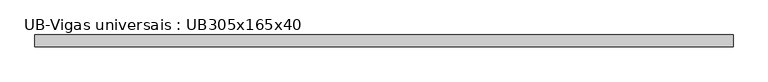
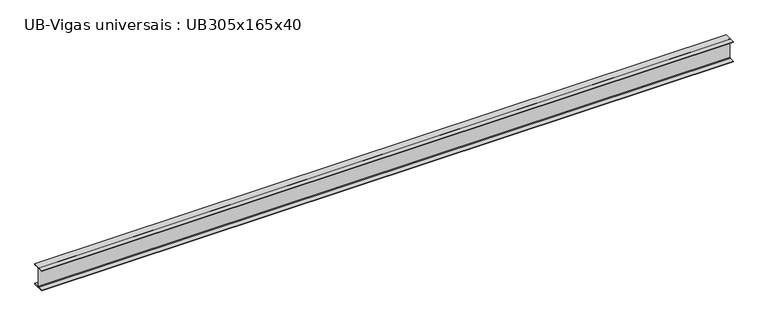
"""IFC4 building model written with IfcOpenShell, lengths in millimetres: beam geometry, UB-Vigas universais : UB305x165x40."""

import ifcopenshell
import ifcopenshell.guid

model = None  # the IFC model being written
_history = None  # IfcOwnerHistory: only IFC2X3 demands one
_inside = {}  # id of a spatial element -> (the spatial element, [elements in it])
_under = {}  # id of a project, library or spatial element -> (it, [spatial elements below it])
_declared = {}  # id of a project -> (the project, [libraries it declares])
_typed = {}  # id of a type object -> (the type object, [elements of that type])
_made_of = {}  # id of a material, layer set ... -> (it, [elements and type objects made of it])


def new_model(schema):
    """Start an empty IFC model of exactly this schema.

    Asked for "IFC4X3", IfcOpenShell would pick the latest addendum, in which some entities
    have other attributes; the version numbers below select the first issue.
    IFC2X3 requires an IfcOwnerHistory on every rooted entity: one is made here for all.
    """
    global model, _history
    if schema == "IFC4X3":
        model = ifcopenshell.file(schema_version=(4, 3, 0, 0))
    else:
        model = ifcopenshell.file(schema=schema)
    _inside.clear()
    _under.clear()
    _declared.clear()
    _typed.clear()
    _made_of.clear()
    _history = None
    if model.schema == "IFC2X3":
        org = make("IfcOrganization", Name="unknown")
        user = make(
            "IfcPersonAndOrganization",
            ThePerson=make("IfcPerson", FamilyName="unknown"),
            TheOrganization=org,
        )
        app = make(
            "IfcApplication",
            ApplicationDeveloper=org,
            Version="unknown",
            ApplicationFullName="unknown",
            ApplicationIdentifier="unknown",
        )
        _history = make(
            "IfcOwnerHistory",
            OwningUser=user,
            OwningApplication=app,
            ChangeAction="ADDED",
            CreationDate=0,
        )
    return model


def make(cls, **values):
    """One entity of the class cls with the attributes given. An attribute that is None is left unset."""
    return model.create_entity(
        cls, **{name: value for name, value in values.items() if value is not None}
    )


def rooted(cls, **values):
    """An entity with a GlobalId (a new one), such as an element, a storey or a relation."""
    return make(cls, GlobalId=ifcopenshell.guid.new(), OwnerHistory=_history, **values)


def si_unit(unit_type, name, prefix=None):
    """IfcSIUnit, for example si_unit("LENGTHUNIT", "METRE", prefix="MILLI")."""
    return make("IfcSIUnit", UnitType=unit_type, Prefix=prefix, Name=name)


def assignment(units):
    """IfcUnitAssignment: the units of a project."""
    return None if units is None else make("IfcUnitAssignment", Units=units)


def point(xyz):
    """IfcCartesianPoint."""
    return None if xyz is None else make("IfcCartesianPoint", Coordinates=xyz)


def direction(xyz):
    """IfcDirection."""
    return None if xyz is None else make("IfcDirection", DirectionRatios=xyz)


def frame(location, z_axis=None, x_axis=None):
    """IfcAxis2Placement3D, a coordinate frame: its origin and axes. An axis left out is left unset."""
    return make(
        "IfcAxis2Placement3D",
        Location=point(location),
        Axis=direction(z_axis),
        RefDirection=direction(x_axis),
    )


def frame_2d(location, x_axis=None):
    """IfcAxis2Placement2D, a coordinate frame in the plane: its origin and x axis."""
    return make(
        "IfcAxis2Placement2D", Location=point(location), RefDirection=direction(x_axis)
    )


def origin():
    """The frame at (0, 0, 0) with its axes left unset."""
    return frame((0.0, 0.0, 0.0))


def place(relative_to, where):
    """IfcLocalPlacement: puts the frame where relative to a parent placement (None: the world)."""
    return make(
        "IfcLocalPlacement", PlacementRelTo=relative_to, RelativePlacement=where
    )


def context(
    kind, dimensions, precision=None, world=None, true_north=None, identifier=None
):
    """IfcGeometricRepresentationContext, for example the 3D "Model" context."""
    return make(
        "IfcGeometricRepresentationContext",
        ContextIdentifier=identifier,
        ContextType=kind,
        CoordinateSpaceDimension=dimensions,
        Precision=precision,
        WorldCoordinateSystem=world,
        TrueNorth=true_north,
    )


def project(units=None, contexts=None):
    """IfcProject with its units and contexts."""
    return rooted(
        "IfcProject",
        Name="project",
        RepresentationContexts=contexts,
        UnitsInContext=assignment(units),
    )


def spatial(cls, under=None, at=None, **own):
    """A site, building, storey or space (cls), placed at a placement, below another one or the project."""
    s = rooted(cls, ObjectPlacement=at, **own)
    if under is not None:
        _under.setdefault(under.id(), (under, []))[1].append(s)
    return s


def polyline(points):
    """IfcPolyline through the points."""
    return make("IfcPolyline", Points=[point(p) for p in points])


def circle_curve(where, radius):
    """IfcCircle in the frame where."""
    return make("IfcCircle", Position=where, Radius=radius)


def trimmed(basis, trim1, trim2, sense, master):
    """IfcTrimmedCurve: the piece of a basis curve between two trims."""
    return make(
        "IfcTrimmedCurve",
        BasisCurve=basis,
        Trim1=trim1,
        Trim2=trim2,
        SenseAgreement=sense,
        MasterRepresentation=master,
    )


def segment(curve, same_sense, transition):
    """IfcCompositeCurveSegment."""
    return make(
        "IfcCompositeCurveSegment",
        Transition=transition,
        SameSense=same_sense,
        ParentCurve=curve,
    )


def composite_curve(segments, self_intersect=None):
    """IfcCompositeCurve: segments joined end to end."""
    return make("IfcCompositeCurve", Segments=segments, SelfIntersect=self_intersect)


def outline(outer, holes=None, kind="AREA"):
    """IfcArbitraryClosedProfileDef: a profile drawn as a closed curve; with holes, ...WithVoids."""
    if holes is None:
        return make("IfcArbitraryClosedProfileDef", ProfileType=kind, OuterCurve=outer)
    return make(
        "IfcArbitraryProfileDefWithVoids",
        ProfileType=kind,
        OuterCurve=outer,
        InnerCurves=holes,
    )


def extrude(swept, where, along, depth):
    """IfcExtrudedAreaSolid: the profile swept, set in the frame where, extruded along a direction by depth."""
    return make(
        "IfcExtrudedAreaSolid",
        SweptArea=swept,
        Position=where,
        ExtrudedDirection=direction(along),
        Depth=depth,
    )


def shape(context_of_items, identifier, shape_type, items):
    """IfcShapeRepresentation: the items that make up one representation, for example the "Body"."""
    return make(
        "IfcShapeRepresentation",
        ContextOfItems=context_of_items,
        RepresentationIdentifier=identifier,
        RepresentationType=shape_type,
        Items=items,
    )


def source(mapping_origin, context_of_items, identifier, shape_type, items):
    """IfcRepresentationMap: a shape defined once, which mapped items show again and again."""
    return make(
        "IfcRepresentationMap",
        MappingOrigin=mapping_origin,
        MappedRepresentation=shape(context_of_items, identifier, shape_type, items),
    )


def transform(
    local_origin,
    x_axis=None,
    y_axis=None,
    z_axis=None,
    scale=None,
    scale2=None,
    scale3=None,
    uniform=True,
):
    """IfcCartesianTransformationOperator3D, or its non-uniform kind. x_axis, y_axis, z_axis: its Axis1, 2, 3."""
    if uniform:
        return make(
            "IfcCartesianTransformationOperator3D",
            Axis1=direction(x_axis),
            Axis2=direction(y_axis),
            LocalOrigin=point(local_origin),
            Scale=scale,
            Axis3=direction(z_axis),
        )
    return make(
        "IfcCartesianTransformationOperator3DnonUniform",
        Axis1=direction(x_axis),
        Axis2=direction(y_axis),
        LocalOrigin=point(local_origin),
        Scale=scale,
        Axis3=direction(z_axis),
        Scale2=scale2,
        Scale3=scale3,
    )


def mapped(mapping_source, mapping_target):
    """IfcMappedItem: shows the shape of a source again, moved by a transform."""
    return make(
        "IfcMappedItem", MappingSource=mapping_source, MappingTarget=mapping_target
    )


def made_of(thing, what):
    """Note that an element or type object is made of a material, layer set ...; save() writes the relation."""
    if what is not None:
        _made_of.setdefault(what.id(), (what, []))[1].append(thing)
    return thing


def element(
    cls,
    number,
    at=None,
    inside=None,
    cuts=None,
    type_object=None,
    material=None,
    context=None,
    identifier="Body",
    shape_type=None,
    held_by="IfcProductDefinitionShape",
    body=None,
    shapes=None,
    **own,
):
    """One element of the class cls, such as IfcWall. Its Tag is "e" and its number.

    at: its placement. inside: the storey or other place that contains it. cuts: it is an
    opening in that element (IfcRelVoidsElement). A single representation is given by context,
    identifier, shape_type and body (its items); several are given by shapes. held_by: the class
    of the entity that holds the representations. save() writes the other relations.
    """
    e = rooted(cls, Tag="e%d" % number, ObjectPlacement=at, **own)
    if body is not None:
        shapes = [shape(context, identifier, shape_type, body)]
    if shapes is not None:
        e.Representation = make(held_by, Representations=shapes)
    if inside is not None:
        _inside.setdefault(inside.id(), (inside, []))[1].append(e)
    if cuts is not None:
        rooted(
            "IfcRelVoidsElement", RelatingBuildingElement=cuts, RelatedOpeningElement=e
        )
    if type_object is not None:
        _typed.setdefault(type_object.id(), (type_object, []))[1].append(e)
    return made_of(e, material)


def aggregate(whole, parts):
    """IfcRelAggregates: a whole, such as a stair, and the parts it consists of."""
    return rooted("IfcRelAggregates", RelatingObject=whole, RelatedObjects=parts)


def save(model, path):
    """Write the relations noted so far, then the file.

    IfcRelAggregates (storeys below a building ...), IfcRelContainedInSpatialStructure (elements
    in a storey), IfcRelDefinesByType, IfcRelAssociatesMaterial and IfcRelDeclares: one each for
    every whole, place, type object, material and project.
    """
    for whole, parts in _under.values():
        aggregate(whole, parts)
    for where, things in _inside.values():
        rooted(
            "IfcRelContainedInSpatialStructure",
            RelatedElements=things,
            RelatingStructure=where,
        )
    for kind, things in _typed.values():
        rooted("IfcRelDefinesByType", RelatedObjects=things, RelatingType=kind)
    for what, things in _made_of.values():
        rooted("IfcRelAssociatesMaterial", RelatedObjects=things, RelatingMaterial=what)
    for by, libraries in _declared.values():
        rooted("IfcRelDeclares", RelatingContext=by, RelatedDefinitions=libraries)
    model.write(path)


def ub_vigas_universais_ub305x165x40_08e43834(model_context):
    return source(origin(), model_context, "Body", "SweptSolid", [
        extrude(outline(composite_curve([segment(polyline([(82.5, -141.5), (82.5, -151.7), (-82.5, -151.7), (-82.5, -141.5), (-11.9, -141.5)]), True, "CONTINUOUS"), segment(trimmed(circle_curve(frame_2d((-11.9, -132.6)), 8.9), [point((-11.9, -141.5))], [point((-3.0, -132.6))], True, "CARTESIAN"), True, "CONTINUOUS"), segment(polyline([(-3.0, -132.6), (-3.0, 132.6)]), True, "CONTINUOUS"), segment(trimmed(circle_curve(frame_2d((-11.9, 132.6)), 8.9), [point((-3.0, 132.6))], [point((-11.9, 141.5))], True, "CARTESIAN"), True, "CONTINUOUS"), segment(polyline([(-11.9, 141.5), (-82.5, 141.5), (-82.5, 151.7), (82.5, 151.7), (82.5, 141.5), (11.9, 141.5)]), True, "CONTINUOUS"), segment(trimmed(circle_curve(frame_2d((11.9, 132.6)), 8.9), [point((11.9, 141.5))], [point((3.0, 132.6))], True, "CARTESIAN"), True, "CONTINUOUS"), segment(polyline([(3.0, 132.6), (3.0, -132.6)]), True, "CONTINUOUS"), segment(trimmed(circle_curve(frame_2d((11.9, -132.6)), 8.9), [point((3.0, -132.6))], [point((11.9, -141.5))], True, "CARTESIAN"), True, "CONTINUOUS"), segment(polyline([(11.9, -141.5), (82.5, -141.5)]), True, "CONTINUOUS")], self_intersect=False)), frame((-4904.8, 0.0, 0.0), z_axis=(1.0, 0.0, 0.0), x_axis=(0.0, 1.0, 0.0)), (0.0, 0.0, 1.0), 9809.6),
    ])


if __name__ == "__main__":
    model = new_model("IFC4")
    model_context = context("Model", 3, world=origin())
    ifc_project = project(units=[si_unit("LENGTHUNIT", "METRE", prefix="MILLI")], contexts=[model_context])
    site = spatial("IfcSite", under=ifc_project)
    building = spatial("IfcBuilding", under=site)
    placement = place(None, origin())
    ub_vigas_universais_ub305x165x40_shape = ub_vigas_universais_ub305x165x40_08e43834(model_context)
    element("IfcBeam", 1, ObjectType="UB-Vigas universais : UB305x165x40", at=placement, inside=building, context=model_context, shape_type="MappedRepresentation", body=[
        mapped(ub_vigas_universais_ub305x165x40_shape, transform((0.0, 0.0, 0.0), x_axis=(1.0, 0.0, 0.0), y_axis=(0.0, 1.0, 0.0), z_axis=(0.0, 0.0, 1.0))),
    ])
    save(model, "model.ifc")

# Revit data of these elements
# Type "UB-Vigas universais : UB305x165x40"
#   Section Name Key = "UB305X165X40"
#   Width = 16.5 cm
#   Web Thickness = 0.6 cm
#   Web Fillet = 0.89 cm
#   Warping Constant = 164000.0 cm⁶
#   Torsional Moment of Inertia = 14.70 cm⁴
#   Section Area = 51.3 cm²
#   Plastic Modulus weak axis = 142.0 cm³
#   Plastic Modulus strong axis = 623.0 cm³
#   Nominal Weight = 40.2999 kgf/m
#   Moment of Inertia weak axis = 764.00 cm⁴
#   Moment of Inertia strong axis = 8503.00 cm⁴
#   Height = 30.34 cm
#   Flange Thickness = 1.02 cm
#   Elastic Modulus weak axis = 92.6 cm³
#   Elastic Modulus strong axis = 560.0 cm³
#   Centroid Vertical = 15.17 cm
#   Centroid Horizontal = 8.25 cm
#   Length [instance default] = 1.50 m
#   Structural Material [instance default] = Metal - Aço 43-275
#   Type Comments = ""
#   Assembly Code = ""
# Element 1 (IfcBeam, "UB-Vigas universais : UB305x165x40")
#   Materials on its faces: "Metal - Aço 43-275"
# Materials
#   "Metal - Aço 43-275": class "Metal", colour RGB 247 247 247, transparency 0, Cost = 0
